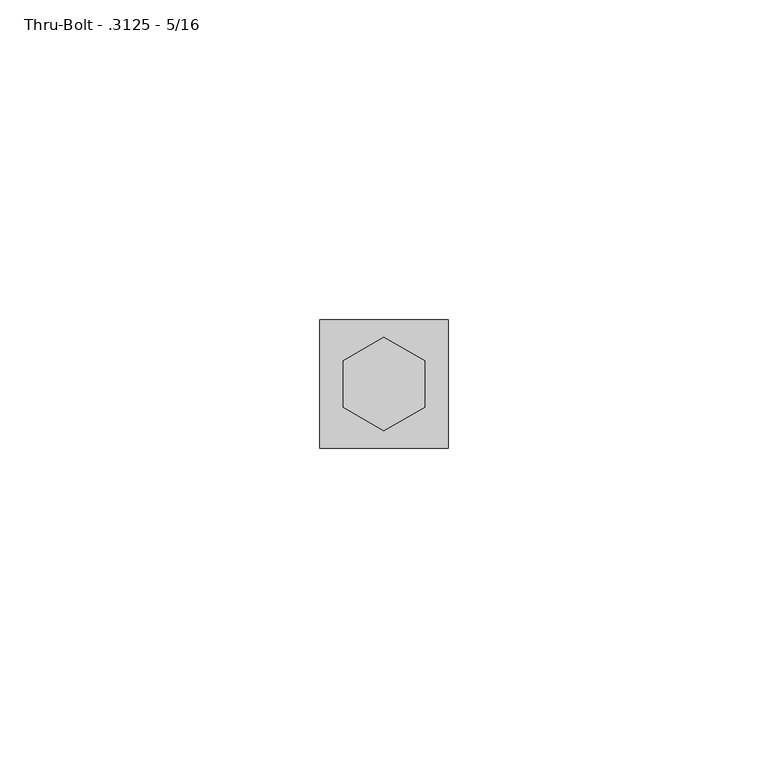
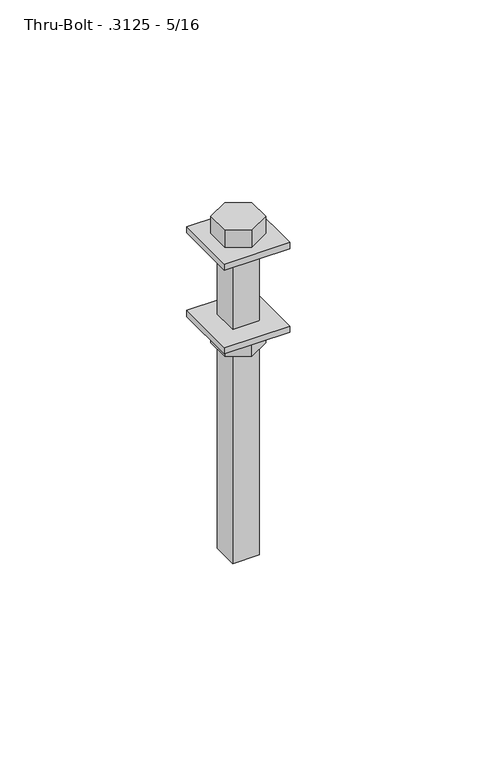
"""IFC4 building model written with IfcOpenShell, lengths in millimetres: fastener geometry, 060523 - W_P_C - Fastenings - Generic - SQUARE : Thru-Bolt - .3125 - 5/16."""

from ifc_helpers import new_model, si_unit, frame, origin, origin_with_axes, place, context, project, spatial, polyline, outline, extrude, source, transform, mapped, element, save


def thru_bolt_3125_5_16_a3b80130(model_context):
    return source(origin(), model_context, "Body", "SweptSolid", [
        extrude(outline(polyline([(-10.067925, -10.067925), (-10.067925, 10.067925), (10.067925, 10.067925), (10.067925, -10.067925), (-10.067925, -10.067925)])), origin_with_axes(), (0.0, 0.0, 1.0), 1.984375),
        extrude(outline(polyline([(-10.067925, -10.067925), (-10.067925, 10.067925), (10.067925, 10.067925), (10.067925, -10.067925), (-10.067925, -10.067925)])), frame((0.0, 0.0, -27.384375), z_axis=(0.0, 0.0, 1.0), x_axis=(1.0, 0.0, 0.0)), (0.0, 0.0, 1.0), 1.984375),
        extrude(outline(polyline([(-6.35, -3.6661742), (-6.35, 3.6661742), (0.0, 7.3323484), (6.35, 3.6661742), (6.35, -3.6661742), (0.0, -7.3323484), (-6.35, -3.6661742)])), frame((0.0, 0.0, -33.3375), z_axis=(0.0, 0.0, 1.0), x_axis=(1.0, 0.0, 0.0)), (0.0, 0.0, 1.0), 5.953125),
        extrude(outline(polyline([(-6.35, 3.6661742), (0.0, 7.3323484), (6.35, 3.6661742), (6.35, -3.6661742), (0.0, -7.3323484), (-6.35, -3.6661742), (-6.35, 3.6661742)])), frame((0.0, 0.0, 1.984375), z_axis=(0.0, 0.0, 1.0), x_axis=(1.0, 0.0, 0.0)), (0.0, 0.0, 1.0), 5.953125),
        extrude(outline(polyline([(-4.1148, 4.1148), (4.1148, 4.1148), (4.1148, -4.1148), (-4.1148, -4.1148), (-4.1148, 4.1148)])), frame((0.0, 0.0, -101.6), z_axis=(0.0, 0.0, 1.0), x_axis=(1.0, 0.0, 0.0)), (0.0, 0.0, 1.0), 103.584375),
    ])


if __name__ == "__main__":
    model = new_model("IFC4")
    model_context = context("Model", 3, world=origin())
    ifc_project = project(units=[si_unit("LENGTHUNIT", "METRE", prefix="MILLI")], contexts=[model_context])
    site = spatial("IfcSite", under=ifc_project)
    building = spatial("IfcBuilding", under=site)
    placement = place(None, origin())
    thru_bolt_3125_5_16_shape = thru_bolt_3125_5_16_a3b80130(model_context)
    element("IfcFastener", 1, ObjectType="060523 - W_P_C - Fastenings - Generic - SQUARE : Thru-Bolt - .3125 - 5/16", at=placement, inside=building, context=model_context, shape_type="MappedRepresentation", body=[
        mapped(thru_bolt_3125_5_16_shape, transform((0.0, 0.0, 0.0), x_axis=(1.0, 0.0, 0.0), y_axis=(0.0, 1.0, 0.0), z_axis=(0.0, 0.0, 1.0))),
    ])
    save(model, "model.ifc")

# Revit data of these elements
# Type "060523 - W_P_C - Fastenings - Generic - SQUARE : Thru-Bolt - .3125 - 5/16"
#   Washer_Thickness = 0' - 0 5/64"
#   Washer Radius = 0' - 0.39638"
#   Washer Offset - Head = 0' - 0 5/64"
#   Washer Offset = 0' - 0 5/64"
#   Thickness_of_Substrate [instance default] = 0' - 1"
#   Side = 0' - 0 37/128"
#   Radius = 0' - 0.162"
#   Length [instance default] = 0' - 4"
#   Head Size = 0' - 0 1/2"
#   Head Radius = 0' - 0 1/4"
#   Head Height = 0' - 0 15/64"
#   Double Diameter = 0' - 0.648"
#   Diameter = 0' - 0.324"
#   Default Elevation = 4' - 0"
#   Washer_Nut_Visibility = yes
#   Washer_Head_Visibility = yes
#   Round_Head_Visibility = no
#   Point Visibility = no
#   Nut_Visibility = yes
#   Hex_Head_Visiblilty = yes
#   Washer Material = none
#   Bolt Material (Size) = AT SILL - FASTENER AT 24" O.C.
# Element 1 (IfcFastener, "060523 - W_P_C - Fastenings - Generic - SQUARE : Thru-Bolt - .3125 - 5/16")
#   Materials on its faces: "AT SILL - FASTENER AT 24\" O.C."
# Materials
#   "AT SILL - FASTENER AT 24\" O.C.": class "Generic", colour RGB 120 120 120, transparency 0, Cost = 0
